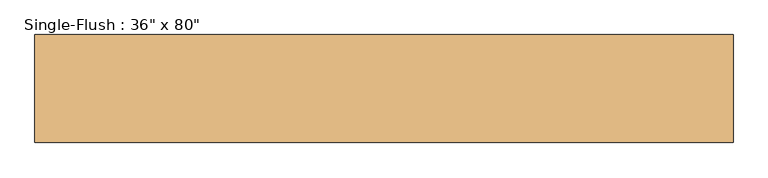
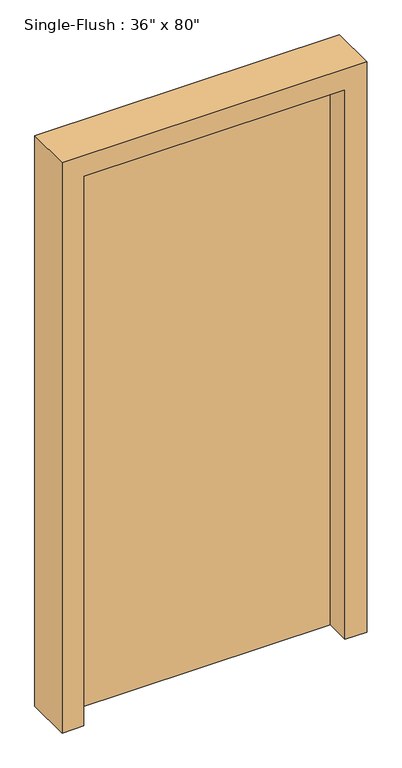
"""IFC4 building model written with IfcOpenShell, lengths in millimetres: door geometry."""

from ifc_helpers import new_model, si_unit, frame, origin, origin_with_axes, place, context, project, spatial, polyline, outline, extrude, source, transform, mapped, element, save


def door_91c1aee8(model_context):
    return source(origin(), model_context, "Body", "SweptSolid", [
        extrude(outline(polyline([(2108.2, 533.4), (2108.2, -533.4), (0.0, -533.4), (0.0, -457.2), (2032.0, -457.2), (2032.0, 457.2), (0.0, 457.2), (0.0, 533.4), (2108.2, 533.4)])), frame((0.0, -82.55, 0.0), z_axis=(0.0, 1.0, 0.0), x_axis=(0.0, 0.0, 1.0)), (0.0, 0.0, 1.0), 165.1),
        extrude(outline(polyline([(457.2, 6.35), (-457.2, 6.35), (-457.2, 57.15), (457.2, 57.15), (457.2, 6.35)])), origin_with_axes(), (0.0, 0.0, 1.0), 2032.0),
    ])


if __name__ == "__main__":
    model = new_model("IFC4")
    model_context = context("Model", 3, world=origin())
    ifc_project = project(units=[si_unit("LENGTHUNIT", "METRE", prefix="MILLI")], contexts=[model_context])
    site = spatial("IfcSite", under=ifc_project)
    building = spatial("IfcBuilding", under=site)
    placement = place(None, origin())
    door_shape = door_91c1aee8(model_context)
    element("IfcDoor", 1, ObjectType="Single-Flush : 36\" x 80\"", at=placement, inside=building, context=model_context, shape_type="MappedRepresentation", body=[
        mapped(door_shape, transform((0.0, 0.0, 0.0), x_axis=(1.0, 0.0, 0.0), y_axis=(0.0, 1.0, 0.0), z_axis=(0.0, 0.0, 1.0))),
    ])
    save(model, "model.ifc")

# Revit data of these elements
# Type "Single-Flush : 36\" x 80\""
#   Type Mark = "6"
#   OD_DS_Door_Material = "T.B.D."
#   OD_DS_Door_Type = "SWING"
#   OD_DS_Lockset = "PRIVACY LOCK"
#   Assembly Code = "C1020"
#   Analytic Construction = "<None>"
#   Thickness = 0' - 2"
#   RO Offset = 0' - 0 1/4"
#   Height = 6' - 8"
#   Trim Projection Ext = 0' - 1"
#   Trim Projection Int = 0' - 1"
#   Trim Width = 0' - 3"
#   Width = 3' - 0"
#   Door Material = Closet_1
#   Frame Material = Closet_1
#   Function = (empty or 0)
#   Wall Closure = (empty or 0)
# Element 1 (IfcDoor, "Single-Flush : 36\" x 80\"")
#   Materials on its faces: "Closet_1"
# Materials
#   "Closet_1": class "Paint", colour RGB 200 194 183, transparency 0, Cost = 0
